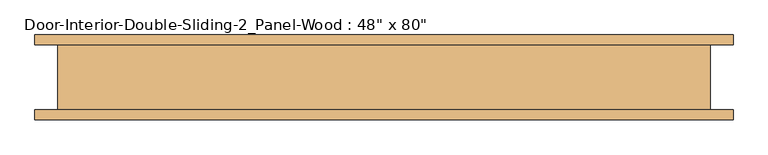
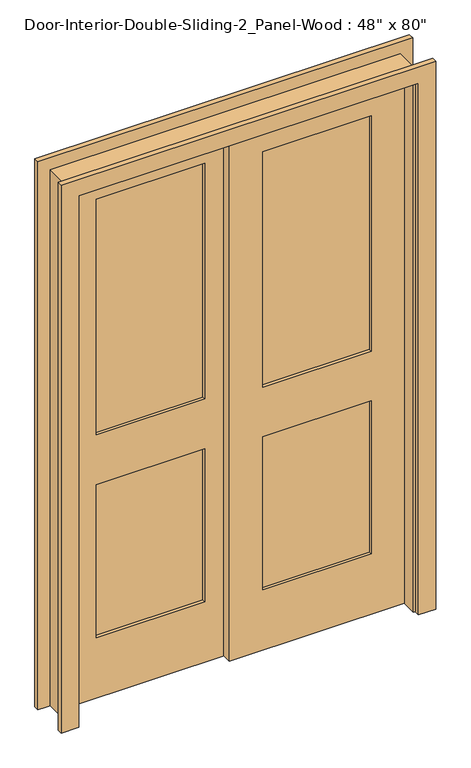
"""IFC4 building model written with IfcOpenShell, lengths in millimetres: door geometry."""

from ifc_helpers import new_model, si_unit, frame, origin, place, context, project, spatial, polyline, outline, extrude, source, transform, mapped, element, save


def door_f5052075(model_context):
    return source(origin(), model_context, "Body", "SweptSolid", [
        extrude(outline(polyline([(488.95, 2.1166667), (95.25, 2.1166667), (95.25, 13.7583333), (488.95, 13.7583333), (488.95, 2.1166667)])), frame((0.0, 0.0, 1009.65), z_axis=(0.0, 0.0, 1.0), x_axis=(1.0, 0.0, 0.0)), (0.0, 0.0, 1.0), 903.2875),
        extrude(outline(polyline([(488.95, 2.1166667), (95.25, 2.1166667), (95.25, 13.7583333), (488.95, 13.7583333), (488.95, 2.1166667)])), frame((0.0, 0.0, 231.775), z_axis=(0.0, 0.0, 1.0), x_axis=(1.0, 0.0, 0.0)), (0.0, 0.0, 1.0), 587.375),
        extrude(outline(polyline([(2032.0, -25.4), (0.0, -25.4), (0.0, 609.6), (2032.0, 609.6), (2032.0, -25.4)]), holes=[polyline([(1912.9375, 95.25), (1912.9375, 488.95), (1009.65, 488.95), (1009.65, 95.25), (1912.9375, 95.25)]), polyline([(819.15, 95.25), (819.15, 488.95), (231.775, 488.95), (231.775, 95.25), (819.15, 95.25)])]), frame((0.0, -9.525, 0.0), z_axis=(0.0, 1.0, 0.0), x_axis=(0.0, 0.0, 1.0)), (0.0, 0.0, 1.0), 34.925),
        extrude(outline(polyline([(-95.25, 37.0416667), (-488.95, 37.0416667), (-488.95, 48.6833333), (-95.25, 48.6833333), (-95.25, 37.0416667)])), frame((0.0, 0.0, 1009.65), z_axis=(0.0, 0.0, 1.0), x_axis=(1.0, 0.0, 0.0)), (0.0, 0.0, 1.0), 903.2875),
        extrude(outline(polyline([(-95.25, 37.0416667), (-488.95, 37.0416667), (-488.95, 48.6833333), (-95.25, 48.6833333), (-95.25, 37.0416667)])), frame((0.0, 0.0, 231.775), z_axis=(0.0, 0.0, 1.0), x_axis=(1.0, 0.0, 0.0)), (0.0, 0.0, 1.0), 587.375),
        extrude(outline(polyline([(2032.0, -609.6), (0.0, -609.6), (0.0, 25.4), (2032.0, 25.4), (2032.0, -609.6)]), holes=[polyline([(1912.9375, -488.95), (1912.9375, -95.25), (1009.65, -95.25), (1009.65, -488.95), (1912.9375, -488.95)]), polyline([(819.15, -488.95), (819.15, -95.25), (231.775, -95.25), (231.775, -488.95), (819.15, -488.95)])]), frame((0.0, 25.4, 0.0), z_axis=(0.0, 1.0, 0.0), x_axis=(0.0, 0.0, 1.0)), (0.0, 0.0, 1.0), 34.925),
        extrude(outline(polyline([(0.0, 609.6), (0.0, 635.0), (2057.4, 635.0), (2057.4, -635.0), (0.0, -635.0), (0.0, -609.6), (2032.0, -609.6), (2032.0, 609.6), (0.0, 609.6)])), frame((0.0, -66.675, 0.0), z_axis=(0.0, 1.0, 0.0), x_axis=(0.0, 0.0, 1.0)), (0.0, 0.0, 1.0), 127.0),
        extrude(outline(polyline([(0.0, 615.95), (0.0, 679.45), (2101.85, 679.45), (2101.85, -679.45), (0.0, -679.45), (0.0, -615.95), (2038.35, -615.95), (2038.35, 615.95), (0.0, 615.95)])), frame((0.0, -85.725, 0.0), z_axis=(0.0, 1.0, 0.0), x_axis=(0.0, 0.0, 1.0)), (0.0, 0.0, 1.0), 19.05),
        extrude(outline(polyline([(0.0, 615.95), (0.0, 679.45), (2101.85, 679.45), (2101.85, -679.45), (0.0, -679.45), (0.0, -615.95), (2038.35, -615.95), (2038.35, 615.95), (0.0, 615.95)])), frame((0.0, 60.325, 0.0), z_axis=(0.0, 1.0, 0.0), x_axis=(0.0, 0.0, 1.0)), (0.0, 0.0, 1.0), 19.05),
    ])


if __name__ == "__main__":
    model = new_model("IFC4")
    model_context = context("Model", 3, world=origin())
    ifc_project = project(units=[si_unit("LENGTHUNIT", "METRE", prefix="MILLI")], contexts=[model_context])
    site = spatial("IfcSite", under=ifc_project)
    building = spatial("IfcBuilding", under=site)
    placement = place(None, origin())
    door_shape = door_f5052075(model_context)
    element("IfcDoor", 1, ObjectType="Door-Interior-Double-Sliding-2_Panel-Wood : 48\" x 80\"", at=placement, inside=building, context=model_context, shape_type="MappedRepresentation", body=[
        mapped(door_shape, transform((0.0, 0.0, 0.0), x_axis=(1.0, 0.0, 0.0), y_axis=(0.0, 1.0, 0.0), z_axis=(0.0, 0.0, 1.0))),
    ])
    save(model, "model.ifc")

# Revit data of these elements
# Type "Door-Interior-Double-Sliding-2_Panel-Wood : 48\" x 80\""
#   Type Mark = "22"
#   Assembly Code = "C1020300"
#   Analytic Construction = "Wooden"
#   Top Rail = 0' - 4 11/16"
#   Thickness = 0' - 1 3/8"
#   Thermal Resistance (R) = 2.5876 (h·ft²·°F)/BTU
#   Stiles = 0' - 4 3/4"
#   Rough Width = 4' - 2"
#   Rough Height = 6' - 9"
#   Lock Rail = 0' - 7 1/2"
#   Height = 6' - 8"
#   Width = 4' - 0"
#   Heat Transfer Coefficient (U) = 0.3865 BTU/(h·ft²·°F)
#   Bottom Rail = 0' - 9 1/8"
#   Trim Material = Cherry
#   Panel Material = Cherry
#   Frame Material = Cherry
#   Visual Light Transmittance = 0
#   Solar Heat Gain Coefficient = 0
#   Wall Closure = (empty or 0)
#   Function = (empty or 0)
# Element 1 (IfcDoor, "Door-Interior-Double-Sliding-2_Panel-Wood : 48\" x 80\"")
#   Materials on its faces: "Cherry"
# Materials
#   "Cherry": class "Wood", colour RGB 226 177 128, transparency 0, Description = "Prunus Serotina", Cost = 0
